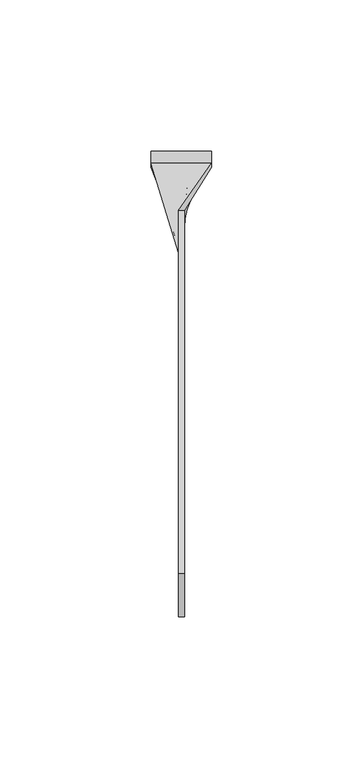
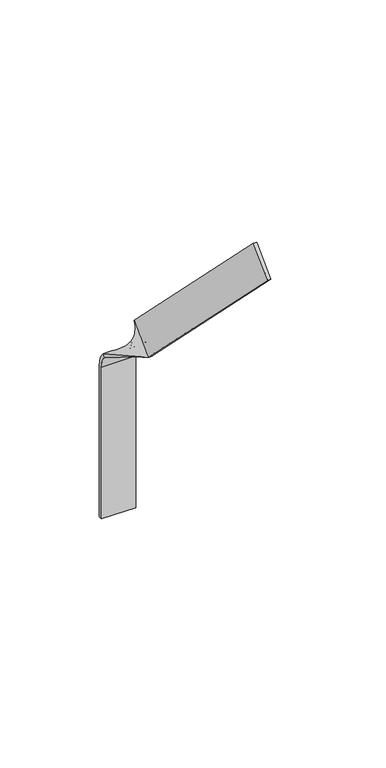
"""IFC4 building model written with IfcOpenShell, lengths in millimetres: proxy geometry, TN_ПВС 125-82_Удлинитель кронштейна боковой : TN_ПВС 125-82_Удлинитель кронштейна боковой."""

from ifc_helpers import new_model, si_unit, frame, origin, place, context, project, spatial, polyline, circle_curve, source, transform, mapped, element, save
from ifc_brep_helpers import plane_surface, cylinder_surface, revolved_surface, spline_surface, advanced_brep


def generic_models_3c4393d3(model_context):
    return source(origin(), model_context, "Body", "AdvancedBrep", [
        advanced_brep(
        [(10.0, -1.8637982, 2.6235265), (-1.0, -17.4320349, 29.4816967), (1.0168115, -17.4320349, 29.4816967), (10.0, -3.2898993, 1.1974254), (-10.0, -1.8637982, 2.6235265), (-1.0, -31.5741705, 15.339561), (-10.0, -3.2898993, 1.1974254), (1.0168115, -31.5741705, 15.339561), (-1.0, -151.7823233, 135.5477138), (1.0168115, -151.7823233, 135.5477138), (1.0168115, -137.6401877, 149.6898495), (-1.0, -137.6401877, 149.6898495), (-10.0, 0.0, -6.7450941), (10.0, 0.0, -6.7450941), (10.0, 2.0168115, -6.7450941), (-10.0, 2.0168115, -6.7450941), (10.0, 0.0, -100.0), (-10.0, 0.0, -100.0), (-10.0, 2.0168115, -100.0), (10.0, 2.0168115, -100.0)],
        [
            (0, 1),
            (1, 2),
            (2, 3),
            (3, 0),
            (0, 4),
            (4, 5),
            (5, 1),
            (4, 6),
            (6, 7),
            (7, 5),
            (2, 7),
            (6, 3),
            (8, 9),
            (9, 10),
            (10, 11),
            (11, 8),
            (11, 1),
            (5, 8),
            (10, 2),
            (9, 7),
            (6, 12, circle_curve(frame((-10.0, -11.2324188, -6.7450941), z_axis=(-1.0, 0.0, 0.0), x_axis=(0.0, 1.0, 0.0)), 11.2324188)),
            (12, 13),
            (13, 3, circle_curve(frame((10.0, -11.2324188, -6.7450941), z_axis=(1.0, 0.0, 0.0), x_axis=(0.0, 1.0, 0.0)), 11.2324188)),
            (0, 14, circle_curve(frame((10.0, -11.2324188, -6.7450941), z_axis=(-1.0, 0.0, 0.0), x_axis=(0.0, 1.0, 0.0)), 13.2492302)),
            (14, 15),
            (15, 4, circle_curve(frame((-10.0, -11.2324188, -6.7450941), z_axis=(1.0, 0.0, 0.0), x_axis=(0.0, 1.0, 0.0)), 13.2492302)),
            (16, 17),
            (17, 18),
            (18, 19),
            (19, 16),
            (12, 17),
            (16, 13),
            (15, 18),
            (14, 19),
        ],
        [
            spline_surface(1, 1, [[(10.0, -3.2898993, 1.1974254), (1.0168115, -17.4320349, 29.4816967)], [(10.0, -1.8637982, 2.6235265), (-1.0, -17.4320349, 29.4816967)]], [2, 2], [2, 2], [0.0, 1.0], [0.0, 1.0]),
            spline_surface(1, 1, [[(10.0, -1.8637982, 2.6235265), (-1.0, -17.4320349, 29.4816967)], [(-10.0, -1.8637982, 2.6235265), (-1.0, -31.5741705, 15.339561)]], [2, 2], [2, 2], [0.0, 1.0], [0.0, 1.0]),
            spline_surface(1, 1, [[(-10.0, -1.8637982, 2.6235265), (-1.0, -31.5741705, 15.339561)], [(-10.0, -3.2898993, 1.1974254), (1.0168115, -31.5741705, 15.339561)]], [2, 2], [2, 2], [0.0, 1.0], [0.0, 1.0]),
            spline_surface(1, 1, [[(-10.0, -3.2898993, 1.1974254), (1.0168115, -31.5741705, 15.339561)], [(10.0, -3.2898993, 1.1974254), (1.0168115, -17.4320349, 29.4816967)]], [2, 2], [2, 2], [0.0, 1.0], [0.0, 1.0]),
            plane_surface(frame((0.0, -144.7112555, 142.6187817), z_axis=(0.0, -0.7071067811865482, 0.707106781186547), x_axis=(1.0, 0.0, 0.0))),
            plane_surface(frame((-1.0, -31.5741705, 15.339561), z_axis=(-1.0000000000000002, 0.0, 0.0), x_axis=(0.0, -0.7071067811865481, 0.707106781186547))),
            plane_surface(frame((-1.0, -17.4320349, 29.4816967), z_axis=(0.0, 0.707106781186547, 0.7071067811865481), x_axis=(0.0, -0.7071067811865481, 0.707106781186547))),
            plane_surface(frame((1.0168115, -17.4320349, 29.4816967), z_axis=(1.0000000000000002, 0.0, 0.0), x_axis=(0.0, -0.7071067811865481, 0.707106781186547))),
            plane_surface(frame((1.0168115, -31.5741705, 15.339561), z_axis=(0.0, -0.707106781186547, -0.7071067811865481), x_axis=(0.0, -0.7071067811865481, 0.707106781186547))),
            revolved_surface(polyline([(10.0, 0.0, -6.7450941), (-10.0, 0.0, -6.7450941)]), (0.0, -11.2324188, -6.7450941), (1.0, 0.0, 0.0)),
            cylinder_surface(frame((0.0, -11.2324188, -6.7450941), z_axis=(1.0, 0.0, 0.0), x_axis=(0.0, 1.0, 0.0)), 13.2492302),
            plane_surface(frame((0.0, 0.0, -100.0), z_axis=(0.0, 0.0, -1.0), x_axis=(1.0, 0.0, 0.0))),
            plane_surface(frame((10.0, 0.0, -100.0), z_axis=(0.0, -1.0, 0.0), x_axis=(0.0, 0.0, 1.0))),
            plane_surface(frame((-10.0, 0.0, -100.0), z_axis=(-1.0, 0.0, 0.0), x_axis=(0.0, 0.0, 1.0))),
            plane_surface(frame((-10.0, 2.0168115, -100.0), z_axis=(0.0, 1.0, 0.0), x_axis=(0.0, 0.0, 1.0))),
            plane_surface(frame((10.0, 2.0168115, -100.0), z_axis=(1.0, 0.0, 0.0), x_axis=(0.0, 0.0, 1.0))),
        ],
        [
            (0, [[1, 2, 3, 4]]),
            (1, [[-1, 5, 6, 7]]),
            (2, [[-6, 8, 9, 10]]),
            (3, [[-3, 11, -9, 12]]),
            (4, [[13, 14, 15, 16]]),
            (5, [[-16, 17, -7, 18]]),
            (6, [[-15, 19, -2, -17]]),
            (7, [[-14, 20, -11, -19]]),
            (8, [[-13, -18, -10, -20]]),
            (9, [[21, 22, 23, -12]]),
            (10, [[24, 25, 26, -5]]),
            (11, [[27, 28, 29, 30]]),
            (12, [[-22, 31, -27, 32]]),
            (13, [[-21, -8, -26, 33, -28, -31]]),
            (14, [[-25, 34, -29, -33]]),
            (15, [[-23, -32, -30, -34, -24, -4]]),
        ],
    ),
    ])


if __name__ == "__main__":
    model = new_model("IFC4")
    model_context = context("Model", 3, world=origin())
    ifc_project = project(units=[si_unit("LENGTHUNIT", "METRE", prefix="MILLI")], contexts=[model_context])
    site = spatial("IfcSite", under=ifc_project)
    building = spatial("IfcBuilding", under=site)
    placement = place(None, origin())
    generic_models_shape = generic_models_3c4393d3(model_context)
    element("IfcBuildingElementProxy", 1, Name="TN_ПВС 125-82_Удлинитель кронштейна боковой : TN_ПВС 125-82_Удлинитель кронштейна боковой", ObjectType="TN_ПВС 125-82_Удлинитель кронштейна боковой : TN_ПВС 125-82_Удлинитель кронштейна боковой", at=placement, inside=building, context=model_context, shape_type="MappedRepresentation", body=[
        mapped(generic_models_shape, transform((0.0, 0.0, 0.0), x_axis=(1.0, 0.0, 0.0), y_axis=(0.0, 1.0, 0.0), z_axis=(0.0, 0.0, 1.0))),
    ])
    save(model, "model.ifc")

# Revit data of these elements
# Type "TN_ПВС 125-82_Удлинитель кронштейна боковой : TN_ПВС 125-82_Удлинитель кронштейна боковой"
#   Description = "Предназначен для крепления кронштейна желоба к стропильной ноге\r\nили на скат крыши"
#   Manufacturer = "ТехноНИКОЛЬ"
#   Model = "Комплектующие к водосточным системам"
#   URL = "https://tn-vodostok.ru/catalog/pvh/"
#   ADSK_Обозначение = "ТехноНИКОЛЬ"
#   ADSK_Наименование краткое = "Удлинитель кронштейна"
#   ADSK_Наименование = "Удлинитель кронштейна боковой"
#   ADSK_Масса_Текст = ""
#   ADSK_Марка = ""
#   ADSK_Код изделия = ""
#   ADSK_Завод-изготовитель = "ТехноНИКОЛЬ"
#   ADSK_Единица измерения = "шт."
#   ADSK_Группирование = "Комплектующие к водосточным системам"
#   ADSK_URL страницы изделия = "https://tn-vodostok.ru/catalog/pvh/"
#   ADSK_URL документации изделия = "https://tn-vodostok.ru/upload/iblock/c42/c427963cb77eb5c3c51f0cfb870e9e52.pdf"
#   ADSK_Размер_Ширина = 20 mm
#   ADSK_Размер_УголПоворота [instance default] = 20.00°
#   ADSK_Размер_Длина [instance default] = 150 mm
#   ADSK_Размер_Высота = 100 mm
#   ADSK_Количество = 1
#   ADSK_Материал = TN_СтальГальванизированная_Серый
#   Default Elevation = 0
# Element 1 (IfcBuildingElementProxy, "TN_ПВС 125-82_Удлинитель кронштейна боковой : TN_ПВС 125-82_Удлинитель кронштейна боковой")
#   ADSK_Размер_УголПоворота = 45.00°
#   ADSK_Размер_Длина = 200 mm
#   Materials on its faces: "TN_СтальГальванизированная_Серый"
# Materials
#   "TN_СтальГальванизированная_Серый": class "Типовые", colour RGB 206 210 213, transparency 0, Cost = 0
